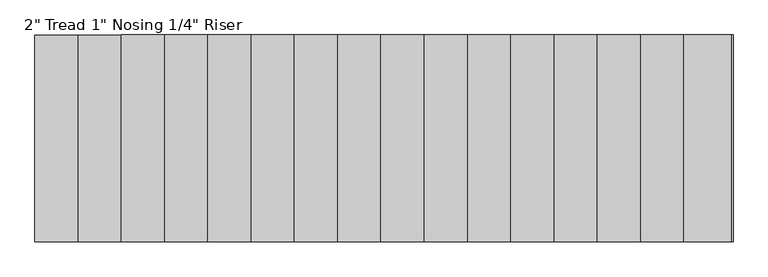
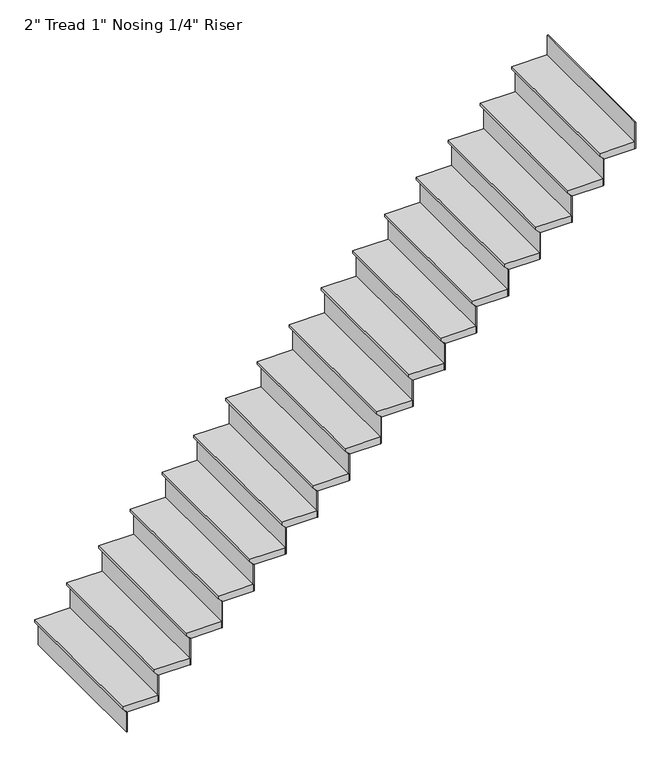
"""IFC4 building model written with IfcOpenShell, lengths in millimetres: stair flight geometry."""

from ifc_helpers import new_model, si_unit, frame, origin, origin_with_axes, place, context, project, spatial, polyline, outline, extrude, source, transform, mapped, element, save


def stair_flight_e7d9a19f(model_context):
    return source(origin(), model_context, "Body", "SweptSolid", [
        extrude(outline(polyline([(200.2117647, 27178.3323402), (200.2117647, 26924.3323402), (181.1617647, 26924.3323402), (155.7617647, 26949.7323402), (149.4117647, 26949.7323402), (149.4117647, 27178.3323402), (200.2117647, 27178.3323402)])), frame((0.0, -15405.5330088, 0.0), z_axis=(0.0, 1.0, 0.0), x_axis=(0.0, 0.0, 1.0)), (0.0, 0.0, 1.0), 1092.2),
        extrude(outline(polyline([(26956.0823402, -15405.5330088), (26949.7323402, -15405.5330088), (26949.7323402, -14313.3330088), (26956.0823402, -14313.3330088), (26956.0823402, -15405.5330088)])), origin_with_axes(), (0.0, 0.0, 1.0), 149.4117647),
        extrude(outline(polyline([(27184.6823402, -15405.5330088), (27178.3323402, -15405.5330088), (27178.3323402, -14313.3330088), (27184.6823402, -14313.3330088), (27184.6823402, -15405.5330088)])), frame((0.0, 0.0, 149.4117647), z_axis=(0.0, 0.0, 1.0), x_axis=(1.0, 0.0, 0.0)), (0.0, 0.0, 1.0), 200.2117647),
        extrude(outline(polyline([(400.4235294, 27406.9323402), (400.4235294, 27152.9323402), (381.3735294, 27152.9323402), (355.9735294, 27178.3323402), (349.6235294, 27178.3323402), (349.6235294, 27406.9323402), (400.4235294, 27406.9323402)])), frame((0.0, -15405.5330088, 0.0), z_axis=(0.0, 1.0, 0.0), x_axis=(0.0, 0.0, 1.0)), (0.0, 0.0, 1.0), 1092.2),
        extrude(outline(polyline([(27413.2823402, -15405.5330088), (27406.9323402, -15405.5330088), (27406.9323402, -14313.3330088), (27413.2823402, -14313.3330088), (27413.2823402, -15405.5330088)])), frame((0.0, 0.0, 349.6235294), z_axis=(0.0, 0.0, 1.0), x_axis=(1.0, 0.0, 0.0)), (0.0, 0.0, 1.0), 200.2117647),
        extrude(outline(polyline([(600.6352941, 27635.5323402), (600.6352941, 27381.5323402), (581.5852941, 27381.5323402), (556.1852941, 27406.9323402), (549.8352941, 27406.9323402), (549.8352941, 27635.5323402), (600.6352941, 27635.5323402)])), frame((0.0, -15405.5330088, 0.0), z_axis=(0.0, 1.0, 0.0), x_axis=(0.0, 0.0, 1.0)), (0.0, 0.0, 1.0), 1092.2),
        extrude(outline(polyline([(27641.8823402, -15405.5330088), (27635.5323402, -15405.5330088), (27635.5323402, -14313.3330088), (27641.8823402, -14313.3330088), (27641.8823402, -15405.5330088)])), frame((0.0, 0.0, 549.8352941), z_axis=(0.0, 0.0, 1.0), x_axis=(1.0, 0.0, 0.0)), (0.0, 0.0, 1.0), 200.2117647),
        extrude(outline(polyline([(800.8470588, 27864.1323402), (800.8470588, 27610.1323402), (781.7970588, 27610.1323402), (756.3970588, 27635.5323402), (750.0470588, 27635.5323402), (750.0470588, 27864.1323402), (800.8470588, 27864.1323402)])), frame((0.0, -15405.5330088, 0.0), z_axis=(0.0, 1.0, 0.0), x_axis=(0.0, 0.0, 1.0)), (0.0, 0.0, 1.0), 1092.2),
        extrude(outline(polyline([(27870.4823402, -15405.5330088), (27864.1323402, -15405.5330088), (27864.1323402, -14313.3330088), (27870.4823402, -14313.3330088), (27870.4823402, -15405.5330088)])), frame((0.0, 0.0, 750.0470588), z_axis=(0.0, 0.0, 1.0), x_axis=(1.0, 0.0, 0.0)), (0.0, 0.0, 1.0), 200.2117647),
        extrude(outline(polyline([(1001.0588235, 28092.7323402), (1001.0588235, 27838.7323402), (982.0088235, 27838.7323402), (956.6088235, 27864.1323402), (950.2588235, 27864.1323402), (950.2588235, 28092.7323402), (1001.0588235, 28092.7323402)])), frame((0.0, -15405.5330088, 0.0), z_axis=(0.0, 1.0, 0.0), x_axis=(0.0, 0.0, 1.0)), (0.0, 0.0, 1.0), 1092.2),
        extrude(outline(polyline([(28099.0823402, -15405.5330088), (28092.7323402, -15405.5330088), (28092.7323402, -14313.3330088), (28099.0823402, -14313.3330088), (28099.0823402, -15405.5330088)])), frame((0.0, 0.0, 950.2588235), z_axis=(0.0, 0.0, 1.0), x_axis=(1.0, 0.0, 0.0)), (0.0, 0.0, 1.0), 200.2117647),
        extrude(outline(polyline([(1201.2705882, 28321.3323402), (1201.2705882, 28067.3323402), (1182.2205882, 28067.3323402), (1156.8205882, 28092.7323402), (1150.4705882, 28092.7323402), (1150.4705882, 28321.3323402), (1201.2705882, 28321.3323402)])), frame((0.0, -15405.5330088, 0.0), z_axis=(0.0, 1.0, 0.0), x_axis=(0.0, 0.0, 1.0)), (0.0, 0.0, 1.0), 1092.2),
        extrude(outline(polyline([(28327.6823402, -15405.5330088), (28321.3323402, -15405.5330088), (28321.3323402, -14313.3330088), (28327.6823402, -14313.3330088), (28327.6823402, -15405.5330088)])), frame((0.0, 0.0, 1150.4705882), z_axis=(0.0, 0.0, 1.0), x_axis=(1.0, 0.0, 0.0)), (0.0, 0.0, 1.0), 200.2117647),
        extrude(outline(polyline([(1401.4823529, 28549.9323402), (1401.4823529, 28295.9323402), (1382.4323529, 28295.9323402), (1357.0323529, 28321.3323402), (1350.6823529, 28321.3323402), (1350.6823529, 28549.9323402), (1401.4823529, 28549.9323402)])), frame((0.0, -15405.5330088, 0.0), z_axis=(0.0, 1.0, 0.0), x_axis=(0.0, 0.0, 1.0)), (0.0, 0.0, 1.0), 1092.2),
        extrude(outline(polyline([(28556.2823402, -15405.5330088), (28549.9323402, -15405.5330088), (28549.9323402, -14313.3330088), (28556.2823402, -14313.3330088), (28556.2823402, -15405.5330088)])), frame((0.0, 0.0, 1350.6823529), z_axis=(0.0, 0.0, 1.0), x_axis=(1.0, 0.0, 0.0)), (0.0, 0.0, 1.0), 200.2117647),
        extrude(outline(polyline([(1601.6941176, 28778.5323402), (1601.6941176, 28524.5323402), (1582.6441176, 28524.5323402), (1557.2441176, 28549.9323402), (1550.8941176, 28549.9323402), (1550.8941176, 28778.5323402), (1601.6941176, 28778.5323402)])), frame((0.0, -15405.5330088, 0.0), z_axis=(0.0, 1.0, 0.0), x_axis=(0.0, 0.0, 1.0)), (0.0, 0.0, 1.0), 1092.2),
        extrude(outline(polyline([(28784.8823402, -15405.5330088), (28778.5323402, -15405.5330088), (28778.5323402, -14313.3330088), (28784.8823402, -14313.3330088), (28784.8823402, -15405.5330088)])), frame((0.0, 0.0, 1550.8941176), z_axis=(0.0, 0.0, 1.0), x_axis=(1.0, 0.0, 0.0)), (0.0, 0.0, 1.0), 200.2117647),
        extrude(outline(polyline([(1801.9058824, 29007.1323402), (1801.9058824, 28753.1323402), (1782.8558824, 28753.1323402), (1757.4558824, 28778.5323402), (1751.1058824, 28778.5323402), (1751.1058824, 29007.1323402), (1801.9058824, 29007.1323402)])), frame((0.0, -15405.5330088, 0.0), z_axis=(0.0, 1.0, 0.0), x_axis=(0.0, 0.0, 1.0)), (0.0, 0.0, 1.0), 1092.2),
        extrude(outline(polyline([(29013.4823402, -15405.5330088), (29007.1323402, -15405.5330088), (29007.1323402, -14313.3330088), (29013.4823402, -14313.3330088), (29013.4823402, -15405.5330088)])), frame((0.0, 0.0, 1751.1058824), z_axis=(0.0, 0.0, 1.0), x_axis=(1.0, 0.0, 0.0)), (0.0, 0.0, 1.0), 200.2117647),
        extrude(outline(polyline([(2002.1176471, 29235.7323402), (2002.1176471, 28981.7323402), (1983.0676471, 28981.7323402), (1957.6676471, 29007.1323402), (1951.3176471, 29007.1323402), (1951.3176471, 29235.7323402), (2002.1176471, 29235.7323402)])), frame((0.0, -15405.5330088, 0.0), z_axis=(0.0, 1.0, 0.0), x_axis=(0.0, 0.0, 1.0)), (0.0, 0.0, 1.0), 1092.2),
        extrude(outline(polyline([(29242.0823402, -15405.5330088), (29235.7323402, -15405.5330088), (29235.7323402, -14313.3330088), (29242.0823402, -14313.3330088), (29242.0823402, -15405.5330088)])), frame((0.0, 0.0, 1951.3176471), z_axis=(0.0, 0.0, 1.0), x_axis=(1.0, 0.0, 0.0)), (0.0, 0.0, 1.0), 200.2117647),
        extrude(outline(polyline([(2202.3294118, 29464.3323402), (2202.3294118, 29210.3323402), (2183.2794118, 29210.3323402), (2157.8794118, 29235.7323402), (2151.5294118, 29235.7323402), (2151.5294118, 29464.3323402), (2202.3294118, 29464.3323402)])), frame((0.0, -15405.5330088, 0.0), z_axis=(0.0, 1.0, 0.0), x_axis=(0.0, 0.0, 1.0)), (0.0, 0.0, 1.0), 1092.2),
        extrude(outline(polyline([(29470.6823402, -15405.5330088), (29464.3323402, -15405.5330088), (29464.3323402, -14313.3330088), (29470.6823402, -14313.3330088), (29470.6823402, -15405.5330088)])), frame((0.0, 0.0, 2151.5294118), z_axis=(0.0, 0.0, 1.0), x_axis=(1.0, 0.0, 0.0)), (0.0, 0.0, 1.0), 200.2117647),
        extrude(outline(polyline([(2402.5411765, 29692.9323402), (2402.5411765, 29438.9323402), (2383.4911765, 29438.9323402), (2358.0911765, 29464.3323402), (2351.7411765, 29464.3323402), (2351.7411765, 29692.9323402), (2402.5411765, 29692.9323402)])), frame((0.0, -15405.5330088, 0.0), z_axis=(0.0, 1.0, 0.0), x_axis=(0.0, 0.0, 1.0)), (0.0, 0.0, 1.0), 1092.2),
        extrude(outline(polyline([(29699.2823402, -15405.5330088), (29692.9323402, -15405.5330088), (29692.9323402, -14313.3330088), (29699.2823402, -14313.3330088), (29699.2823402, -15405.5330088)])), frame((0.0, 0.0, 2351.7411765), z_axis=(0.0, 0.0, 1.0), x_axis=(1.0, 0.0, 0.0)), (0.0, 0.0, 1.0), 200.2117647),
        extrude(outline(polyline([(2602.7529412, 29921.5323402), (2602.7529412, 29667.5323402), (2583.7029412, 29667.5323402), (2558.3029412, 29692.9323402), (2551.9529412, 29692.9323402), (2551.9529412, 29921.5323402), (2602.7529412, 29921.5323402)])), frame((0.0, -15405.5330088, 0.0), z_axis=(0.0, 1.0, 0.0), x_axis=(0.0, 0.0, 1.0)), (0.0, 0.0, 1.0), 1092.2),
        extrude(outline(polyline([(29927.8823402, -15405.5330088), (29921.5323402, -15405.5330088), (29921.5323402, -14313.3330088), (29927.8823402, -14313.3330088), (29927.8823402, -15405.5330088)])), frame((0.0, 0.0, 2551.9529412), z_axis=(0.0, 0.0, 1.0), x_axis=(1.0, 0.0, 0.0)), (0.0, 0.0, 1.0), 200.2117647),
        extrude(outline(polyline([(2802.9647059, 30150.1323402), (2802.9647059, 29896.1323402), (2783.9147059, 29896.1323402), (2758.5147059, 29921.5323402), (2752.1647059, 29921.5323402), (2752.1647059, 30150.1323402), (2802.9647059, 30150.1323402)])), frame((0.0, -15405.5330088, 0.0), z_axis=(0.0, 1.0, 0.0), x_axis=(0.0, 0.0, 1.0)), (0.0, 0.0, 1.0), 1092.2),
        extrude(outline(polyline([(30156.4823402, -15405.5330088), (30150.1323402, -15405.5330088), (30150.1323402, -14313.3330088), (30156.4823402, -14313.3330088), (30156.4823402, -15405.5330088)])), frame((0.0, 0.0, 2752.1647059), z_axis=(0.0, 0.0, 1.0), x_axis=(1.0, 0.0, 0.0)), (0.0, 0.0, 1.0), 200.2117647),
        extrude(outline(polyline([(3003.1764706, 30378.7323402), (3003.1764706, 30124.7323402), (2984.1264706, 30124.7323402), (2958.7264706, 30150.1323402), (2952.3764706, 30150.1323402), (2952.3764706, 30378.7323402), (3003.1764706, 30378.7323402)])), frame((0.0, -15405.5330088, 0.0), z_axis=(0.0, 1.0, 0.0), x_axis=(0.0, 0.0, 1.0)), (0.0, 0.0, 1.0), 1092.2),
        extrude(outline(polyline([(30385.0823402, -15405.5330088), (30378.7323402, -15405.5330088), (30378.7323402, -14313.3330088), (30385.0823402, -14313.3330088), (30385.0823402, -15405.5330088)])), frame((0.0, 0.0, 2952.3764706), z_axis=(0.0, 0.0, 1.0), x_axis=(1.0, 0.0, 0.0)), (0.0, 0.0, 1.0), 200.2117647),
        extrude(outline(polyline([(30613.6823402, -15405.5330088), (30607.3323402, -15405.5330088), (30607.3323402, -14313.3330088), (30613.6823402, -14313.3330088), (30613.6823402, -15405.5330088)])), frame((0.0, 0.0, 3152.5882353), z_axis=(0.0, 0.0, 1.0), x_axis=(1.0, 0.0, 0.0)), (0.0, 0.0, 1.0), 200.2117647),
        extrude(outline(polyline([(3203.3882353, 30607.3323402), (3203.3882353, 30353.3323402), (3184.3382353, 30353.3323402), (3158.9382353, 30378.7323402), (3152.5882353, 30378.7323402), (3152.5882353, 30607.3323402), (3203.3882353, 30607.3323402)])), frame((0.0, -15405.5330088, 0.0), z_axis=(0.0, 1.0, 0.0), x_axis=(0.0, 0.0, 1.0)), (0.0, 0.0, 1.0), 1092.2),
    ])


if __name__ == "__main__":
    model = new_model("IFC4")
    model_context = context("Model", 3, world=origin())
    ifc_project = project(units=[si_unit("LENGTHUNIT", "METRE", prefix="MILLI")], contexts=[model_context])
    site = spatial("IfcSite", under=ifc_project)
    building = spatial("IfcBuilding", under=site)
    placement = place(None, origin())
    stair_flight_shape = stair_flight_e7d9a19f(model_context)
    element("IfcStairFlight", 1, ObjectType="2\" Tread 1\" Nosing 1/4\" Riser", at=placement, inside=building, context=model_context, shape_type="MappedRepresentation", body=[
        mapped(stair_flight_shape, transform((0.0, 0.0, 0.0), x_axis=(1.0, 0.0, 0.0), y_axis=(0.0, 1.0, 0.0), z_axis=(0.0, 0.0, 1.0))),
    ])
    save(model, "model.ifc")

# Revit data of these elements
# Element 1 (IfcStairFlight, "2\" Tread 1\" Nosing 1/4\" Riser")
#   Materials on its faces: "Default Floor"
# Materials
#   "Default Floor": class "Miscellaneous", colour RGB 255 255 255, transparency 0, Cost = 0
